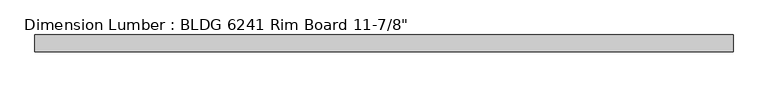
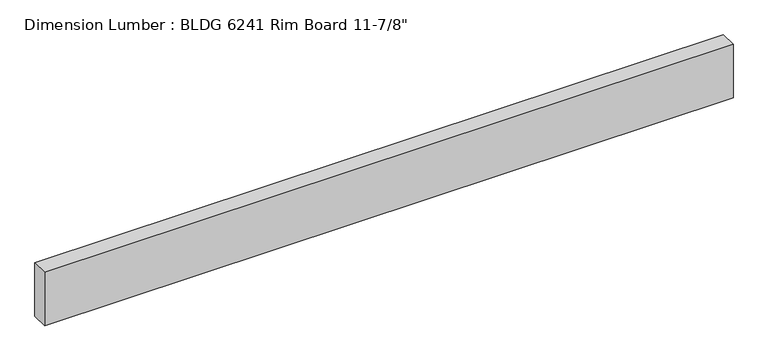
"""IFC4 building model written with IfcOpenShell, lengths in millimetres: beam geometry."""

from ifc_helpers import new_model, si_unit, frame, origin, place, context, project, spatial, polyline, outline, extrude, source, transform, mapped, element, save


def beam_28985cd7(model_context):
    return source(origin(), model_context, "Body", "SweptSolid", [
        extrude(outline(polyline([(1882.775, 44.45), (1882.775, -44.45), (-1793.875, -44.45), (-1793.875, 44.45), (1882.775, 44.45)])), frame((0.0, 0.0, -150.8125), z_axis=(0.0, 0.0, 1.0), x_axis=(1.0, 0.0, 0.0)), (0.0, 0.0, 1.0), 301.625),
    ])


if __name__ == "__main__":
    model = new_model("IFC4")
    model_context = context("Model", 3, world=origin())
    ifc_project = project(units=[si_unit("LENGTHUNIT", "METRE", prefix="MILLI")], contexts=[model_context])
    site = spatial("IfcSite", under=ifc_project)
    building = spatial("IfcBuilding", under=site)
    placement = place(None, origin())
    beam_shape = beam_28985cd7(model_context)
    element("IfcBeam", 1, ObjectType="Dimension Lumber : BLDG 6241 Rim Board 11-7/8\"", at=placement, inside=building, context=model_context, shape_type="MappedRepresentation", body=[
        mapped(beam_shape, transform((0.0, 0.0, 0.0), x_axis=(1.0, 0.0, 0.0), y_axis=(0.0, 1.0, 0.0), z_axis=(0.0, 0.0, 1.0))),
    ])
    save(model, "model.ifc")

# Revit data of these elements
# Type "Dimension Lumber : BLDG 6241 Rim Board 11-7/8\""
#   Assembly Code = "B10"
#   A = 0.273472 SF
#   Length [instance default] = 5' - 0"
#   b = 0' - 3 1/2"
#   d = 0' - 11 7/8"
#   Structural Material [instance default] = Softwood, Lumber
# Element 1 (IfcBeam, "Dimension Lumber : BLDG 6241 Rim Board 11-7/8\"")
#   Materials on its faces: "Softwood, Lumber"
# Materials
#   "Softwood, Lumber": class "Wood", colour RGB 223 192 134, transparency 0, Description = "Pinus Echinata", Cost = 0
